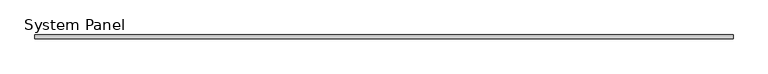
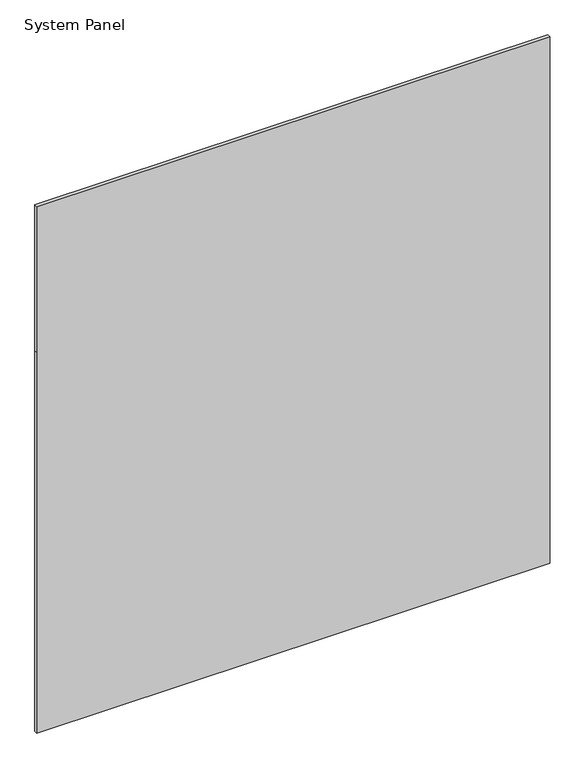
"""IFC4 building model written with IfcOpenShell, lengths in millimetres: plate geometry, System Panel : 로이복층유리_16."""

from ifc_helpers import new_model, si_unit, frame, origin, place, context, project, spatial, polyline, outline, extrude, source, transform, mapped, element, save


def system_panel_f97bc02c(model_context):
    return source(origin(), model_context, "Body", "SweptSolid", [
        extrude(outline(polyline([(0.0, -1388.5), (0.0, 1388.5), (2177.5, 1388.5), (3010.0, 1388.5), (3010.0, -1388.5), (2177.5, -1388.5), (0.0, -1388.5)])), frame((0.0, -8.0, 0.0), z_axis=(0.0, 1.0, 0.0), x_axis=(0.0, 0.0, 1.0)), (0.0, 0.0, 1.0), 16.0),
    ])


if __name__ == "__main__":
    model = new_model("IFC4")
    model_context = context("Model", 3, world=origin())
    ifc_project = project(units=[si_unit("LENGTHUNIT", "METRE", prefix="MILLI")], contexts=[model_context])
    site = spatial("IfcSite", under=ifc_project)
    building = spatial("IfcBuilding", under=site)
    placement = place(None, origin())
    system_panel_shape = system_panel_f97bc02c(model_context)
    element("IfcPlate", 1, ObjectType="System Panel : 로이복층유리_16", at=placement, inside=building, context=model_context, shape_type="MappedRepresentation", body=[
        mapped(system_panel_shape, transform((0.0, 0.0, 0.0), x_axis=(1.0, 0.0, 0.0), y_axis=(0.0, 1.0, 0.0), z_axis=(0.0, 0.0, 1.0))),
    ])
    save(model, "model.ifc")

# Revit data of these elements
# Element 1 (IfcPlate, "System Panel : 로이복층유리_16")
#   Materials on its faces: "00_Glass_Glass"
# Materials
#   "00_Glass_Glass": class "Glass", colour RGB 218 227 224, transparency 0.85, Description = "Glass", Cost = 0, Image = none
